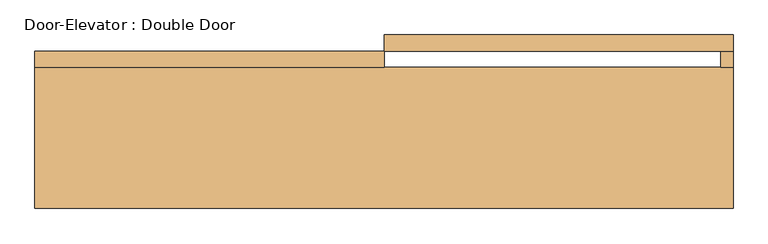
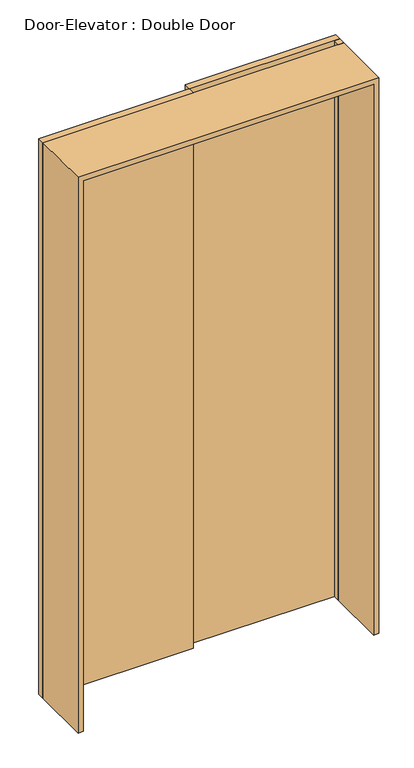
"""IFC4 building model written with IfcOpenShell, lengths in millimetres: door geometry, Door-Elevator : Double Door."""

from ifc_helpers import new_model, si_unit, frame, origin, origin_with_axes, place, context, project, spatial, polyline, outline, extrude, source, transform, mapped, element, save


def door_elevator_double_door_1168a1c9(model_context):
    return source(origin(), model_context, "Body", "SweptSolid", [
        extrude(outline(polyline([(546.1, 157.15), (0.0, 157.15), (0.0, 182.55), (546.1, 182.55), (546.1, 157.15)])), origin_with_axes(), (0.0, 0.0, 1.0), 2133.6),
        extrude(outline(polyline([(0.0, 131.75), (-546.1, 131.75), (-546.1, 157.15), (0.0, 157.15), (0.0, 131.75)])), origin_with_axes(), (0.0, 0.0, 1.0), 2133.6),
        extrude(outline(polyline([(546.1, 131.75), (527.05, 131.75), (527.05, 157.15), (546.1, 157.15), (546.1, 131.75)])), origin_with_axes(), (0.0, 0.0, 1.0), 2133.6),
        extrude(outline(polyline([(0.0, -546.1), (0.0, -527.05), (2114.55, -527.05), (2114.55, 527.05), (0.0, 527.05), (0.0, 546.1), (2133.6, 546.1), (2133.6, -546.1), (0.0, -546.1)])), frame((0.0, -88.9, 0.0), z_axis=(0.0, 1.0, 0.0), x_axis=(0.0, 0.0, 1.0)), (0.0, 0.0, 1.0), 220.65),
    ])


if __name__ == "__main__":
    model = new_model("IFC4")
    model_context = context("Model", 3, world=origin())
    ifc_project = project(units=[si_unit("LENGTHUNIT", "METRE", prefix="MILLI")], contexts=[model_context])
    site = spatial("IfcSite", under=ifc_project)
    building = spatial("IfcBuilding", under=site)
    placement = place(None, origin())
    door_elevator_double_door_shape = door_elevator_double_door_1168a1c9(model_context)
    element("IfcDoor", 1, ObjectType="Door-Elevator : Double Door", at=placement, inside=building, context=model_context, shape_type="MappedRepresentation", body=[
        mapped(door_elevator_double_door_shape, transform((0.0, 0.0, 0.0), x_axis=(1.0, 0.0, 0.0), y_axis=(0.0, 1.0, 0.0), z_axis=(0.0, 0.0, 1.0))),
    ])
    save(model, "model.ifc")

# Revit data of these elements
# Type "Door-Elevator : Double Door"
#   Type Mark = "EX5-"
#   P_WWSKU = ""
#   Filter Visibiilty = "Existing Elevator"
#   Analytic Construction = "<None>"
#   Trim Projection = 12.7 mm
#   Thickness = 25.4 mm
#   Height = 2133.6 mm
#   Trim Width = 19.05 mm
#   Width = 1092.2 mm
#   Door_Quad = 273.05 mm
#   Door_Double = 546.1 mm
#   Cab Width = 1828.8 mm
#   Cab Offset [instance default] = 0 mm
#   Cab Depth = 1828.8 mm
#   _factor4 = 4
#   _factor2 = 2
#   WW-HardwareSet [instance default] = 0
#   Simple Plan = yes
#   Quad = no
#   Plan Lines [instance default] = yes
#   Double = yes
#   Panel Type = element 9002524
#   Type Comments = ""
#   Keynote = ""
#   Function = (empty or 0)
#   Wall Closure = (empty or 0)
#   Assembly Code = ""
# Element 1 (IfcDoor, "Door-Elevator : Double Door")
#   Materials on its faces: "WW-EC-RGB-White"
# Materials
#   "WW-EC-RGB-White": class "Generic", colour RGB 255 255 255, transparency 0, Comments = "If region requests off-white, swith asset color to RGB 231-228-220", Description = "Generic Color", Cost = 0
